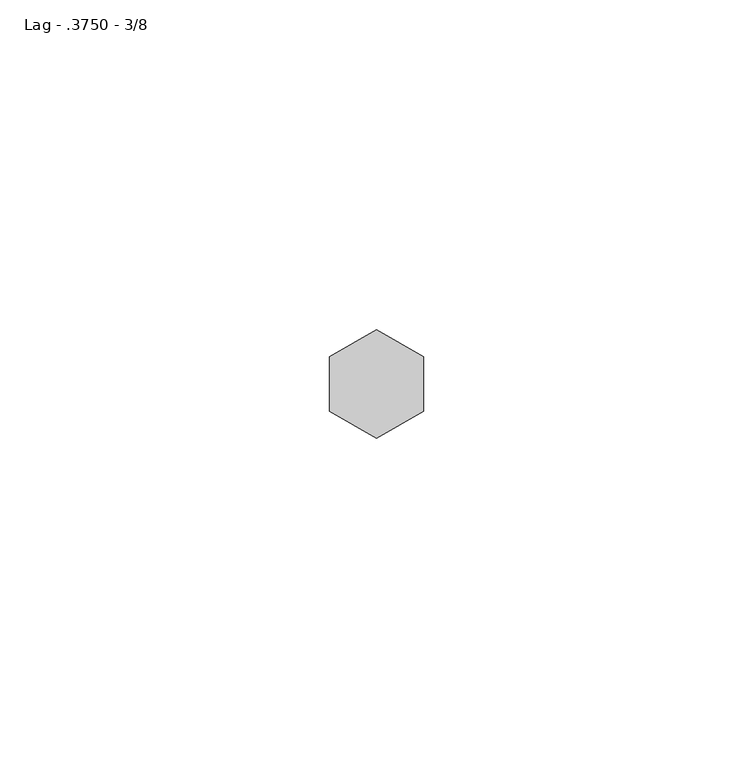
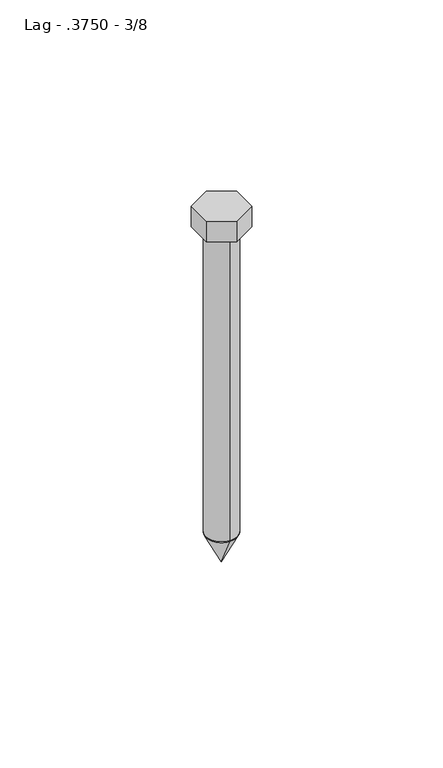
"""IFC4 building model written with IfcOpenShell, lengths in millimetres: fastener geometry, 060523 - W_P_C - Fastenings - Generic : Lag - .3750 - 3/8."""

from ifc_helpers import new_model, si_unit, point, frame, origin, origin_with_axes, origin_2d, place, context, project, spatial, polyline, circle_curve, trimmed, segment, composite_curve, outline, extrude, source, transform, mapped, element, save
from ifc_brep_helpers import plane_surface, revolved_surface, advanced_brep


def lag_3750_3_8_d5ffdfca(model_context):
    return source(origin(), model_context, "Body", "SolidModel", [
        advanced_brep(
        [(0.0, -4.9113281, -101.6), (0.0, 4.9113281, -101.6), (0.0, 0.0, -101.6), (0.0, 0.0, -111.4226562)],
        [
            (0, 1, circle_curve(frame((0.0, 0.0, -101.6), z_axis=(0.0, 0.0, 1.0), x_axis=(0.0, 1.0, 0.0)), 4.9113281)),
            (1, 2),
            (2, 0),
            (1, 0, circle_curve(frame((0.0, 0.0, -101.6), z_axis=(0.0, 0.0, 1.0), x_axis=(0.0, 1.0, 0.0)), 4.9113281)),
            (3, 1),
            (0, 3),
        ],
        [
            plane_surface(frame((0.0, 0.0, -101.6), z_axis=(0.0, 0.0, 1.0), x_axis=(0.0, 1.0, 0.0))),
            revolved_surface(polyline([(0.0, 4.9113281, -101.6), (0.0, 0.0, -111.4226562)]), (0.0, 0.0, -103.0840259), (0.0, 0.0, -1.0)),
        ],
        [
            (0, [[1, 2, 3]]),
            (0, [[4, -3, -2]]),
            (1, [[5, -1, 6]]),
            (1, [[-6, -4, -5]]),
        ],
    ),
        extrude(outline(polyline([(-7.14375, 4.124446), (0.0, 8.248892), (7.14375, 4.124446), (7.14375, -4.124446), (0.0, -8.248892), (-7.14375, -4.124446), (-7.14375, 4.124446)])), origin_with_axes(), (0.0, 0.0, 1.0), 6.8072),
        extrude(outline(composite_curve([segment(trimmed(circle_curve(origin_2d(), 4.9113281), [point((0.0, -4.9113281))], [point((0.0, 4.9113281))], False, "CARTESIAN"), True, "CONTINUOUS"), segment(trimmed(circle_curve(origin_2d(), 4.9113281), [point((0.0, 4.9113281))], [point((0.0, -4.9113281))], False, "CARTESIAN"), True, "CONTINUOUS")], self_intersect=False)), frame((0.0, 0.0, -101.6), z_axis=(0.0, 0.0, 1.0), x_axis=(1.0, 0.0, 0.0)), (0.0, 0.0, 1.0), 101.6),
    ])


if __name__ == "__main__":
    model = new_model("IFC4")
    model_context = context("Model", 3, world=origin())
    ifc_project = project(units=[si_unit("LENGTHUNIT", "METRE", prefix="MILLI")], contexts=[model_context])
    site = spatial("IfcSite", under=ifc_project)
    building = spatial("IfcBuilding", under=site)
    placement = place(None, origin())
    lag_3750_3_8_shape = lag_3750_3_8_d5ffdfca(model_context)
    element("IfcFastener", 1, ObjectType="060523 - W_P_C - Fastenings - Generic : Lag - .3750 - 3/8", at=placement, inside=building, context=model_context, shape_type="MappedRepresentation", body=[
        mapped(lag_3750_3_8_shape, transform((0.0, 0.0, 0.0), x_axis=(1.0, 0.0, 0.0), y_axis=(0.0, 1.0, 0.0), z_axis=(0.0, 0.0, 1.0))),
    ])
    save(model, "model.ifc")

# Revit data of these elements
# Type "060523 - W_P_C - Fastenings - Generic : Lag - .3750 - 3/8"
#   Washer_Thickness = 0' - 0.08933"
#   Washer Radius = 0' - 0.46136"
#   Washer Offset - Head = 0' - 0"
#   Washer Offset = 0' - 0"
#   Thickness_of_Substrate [instance default] = 0' - 1"
#   Side = 0' - 0.3252"
#   Radius = 0' - 0.19336"
#   Length [instance default] = 0' - 4"
#   Head Size = 0' - 0 9/16"
#   Head Radius = 0' - 0 9/32"
#   Head Height = 0' - 0.268"
#   Double Diameter = 0' - 0 99/128"
#   Diameter = 0' - 0 99/256"
#   Default Elevation = 4' - 0"
#   Washer_Nut_Visibility = no
#   Washer_Head_Visibility = no
#   Round_Head_Visibility = no
#   Point Visibility = yes
#   Nut_Visibility = no
#   Hex_Head_Visiblilty = yes
#   Washer Material = none
#   Bolt Material (Size) = AT SILL - FASTENER AT 24" O.C.
# Element 1 (IfcFastener, "060523 - W_P_C - Fastenings - Generic : Lag - .3750 - 3/8")
#   Materials on its faces: "AT SILL - FASTENER AT 24\" O.C."
# Materials
#   "AT SILL - FASTENER AT 24\" O.C.": class "Generic", colour RGB 120 120 120, transparency 0, Cost = 0
